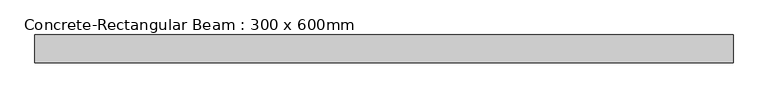
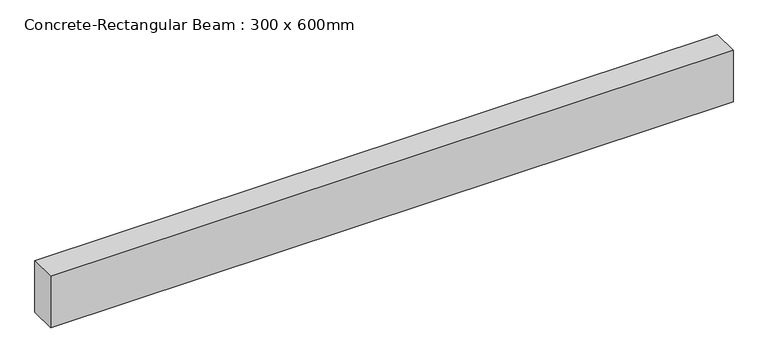
"""IFC4 building model written with IfcOpenShell, lengths in millimetres: beam geometry, Concrete-Rectangular Beam : 300 x 600mm."""

from ifc_helpers import new_model, si_unit, frame, origin, place, context, project, spatial, polyline, outline, extrude, source, transform, mapped, element, save


def concrete_rectangular_beam_300_x_600mm_07bb940a(model_context):
    return source(origin(), model_context, "Body", "SweptSolid", [
        extrude(outline(polyline([(3784.507894, 150.0), (3784.507894, -150.0), (-3784.507894, -150.0), (-3784.507894, 150.0), (3784.507894, 150.0)])), frame((0.0, 0.0, -300.0), z_axis=(0.0, 0.0, 1.0), x_axis=(1.0, 0.0, 0.0)), (0.0, 0.0, 1.0), 600.0),
    ])


if __name__ == "__main__":
    model = new_model("IFC4")
    model_context = context("Model", 3, world=origin())
    ifc_project = project(units=[si_unit("LENGTHUNIT", "METRE", prefix="MILLI")], contexts=[model_context])
    site = spatial("IfcSite", under=ifc_project)
    building = spatial("IfcBuilding", under=site)
    placement = place(None, origin())
    concrete_rectangular_beam_300_x_600mm_shape = concrete_rectangular_beam_300_x_600mm_07bb940a(model_context)
    element("IfcBeam", 1, ObjectType="Concrete-Rectangular Beam : 300 x 600mm", at=placement, inside=building, context=model_context, shape_type="MappedRepresentation", body=[
        mapped(concrete_rectangular_beam_300_x_600mm_shape, transform((0.0, 0.0, 0.0), x_axis=(1.0, 0.0, 0.0), y_axis=(0.0, 1.0, 0.0), z_axis=(0.0, 0.0, 1.0))),
    ])
    save(model, "model.ifc")

# Revit data of these elements
# Type "Concrete-Rectangular Beam : 300 x 600mm"
#   Length [instance default] = 1524 mm
#   b = 300 mm
#   h = 600 mm
#   Structural Material [instance default] = Concrete, Cast-in-Place gray
#   Assembly Code = ""
# Element 1 (IfcBeam, "Concrete-Rectangular Beam : 300 x 600mm")
#   Materials on its faces: "Concrete, Cast-in-Place gray"
# Materials
#   "Concrete, Cast-in-Place gray": class "Concrete", colour RGB 192 192 192, transparency 0, Description = "Cast-in-place concrete", Cost = 0
